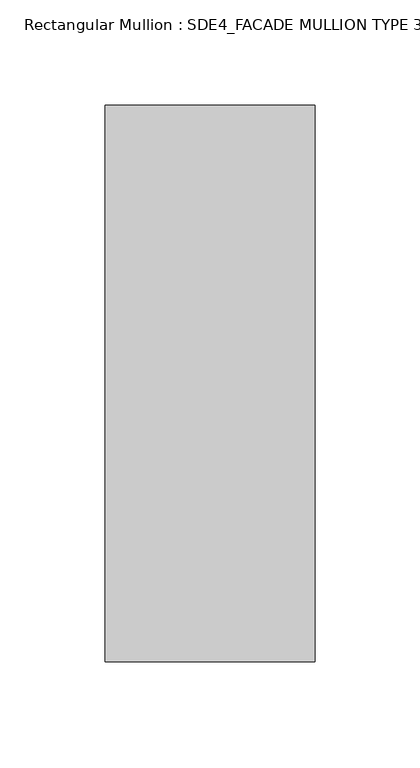
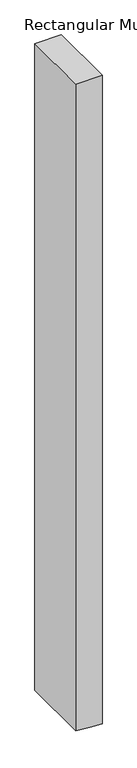
"""IFC4 building model written with IfcOpenShell, lengths in millimetres: member geometry, Rectangular Mullion : SDE4_FACADE MULLION TYPE 3."""

import ifcopenshell
import ifcopenshell.guid

model = None  # the IFC model being written
_history = None  # IfcOwnerHistory: only IFC2X3 demands one
_inside = {}  # id of a spatial element -> (the spatial element, [elements in it])
_under = {}  # id of a project, library or spatial element -> (it, [spatial elements below it])
_declared = {}  # id of a project -> (the project, [libraries it declares])
_typed = {}  # id of a type object -> (the type object, [elements of that type])
_made_of = {}  # id of a material, layer set ... -> (it, [elements and type objects made of it])


def new_model(schema):
    """Start an empty IFC model of exactly this schema.

    Asked for "IFC4X3", IfcOpenShell would pick the latest addendum, in which some entities
    have other attributes; the version numbers below select the first issue.
    IFC2X3 requires an IfcOwnerHistory on every rooted entity: one is made here for all.
    """
    global model, _history
    if schema == "IFC4X3":
        model = ifcopenshell.file(schema_version=(4, 3, 0, 0))
    else:
        model = ifcopenshell.file(schema=schema)
    _inside.clear()
    _under.clear()
    _declared.clear()
    _typed.clear()
    _made_of.clear()
    _history = None
    if model.schema == "IFC2X3":
        org = make("IfcOrganization", Name="unknown")
        user = make(
            "IfcPersonAndOrganization",
            ThePerson=make("IfcPerson", FamilyName="unknown"),
            TheOrganization=org,
        )
        app = make(
            "IfcApplication",
            ApplicationDeveloper=org,
            Version="unknown",
            ApplicationFullName="unknown",
            ApplicationIdentifier="unknown",
        )
        _history = make(
            "IfcOwnerHistory",
            OwningUser=user,
            OwningApplication=app,
            ChangeAction="ADDED",
            CreationDate=0,
        )
    return model


def make(cls, **values):
    """One entity of the class cls with the attributes given. An attribute that is None is left unset."""
    return model.create_entity(
        cls, **{name: value for name, value in values.items() if value is not None}
    )


def rooted(cls, **values):
    """An entity with a GlobalId (a new one), such as an element, a storey or a relation."""
    return make(cls, GlobalId=ifcopenshell.guid.new(), OwnerHistory=_history, **values)


def si_unit(unit_type, name, prefix=None):
    """IfcSIUnit, for example si_unit("LENGTHUNIT", "METRE", prefix="MILLI")."""
    return make("IfcSIUnit", UnitType=unit_type, Prefix=prefix, Name=name)


def assignment(units):
    """IfcUnitAssignment: the units of a project."""
    return None if units is None else make("IfcUnitAssignment", Units=units)


def point(xyz):
    """IfcCartesianPoint."""
    return None if xyz is None else make("IfcCartesianPoint", Coordinates=xyz)


def direction(xyz):
    """IfcDirection."""
    return None if xyz is None else make("IfcDirection", DirectionRatios=xyz)


def frame(location, z_axis=None, x_axis=None):
    """IfcAxis2Placement3D, a coordinate frame: its origin and axes. An axis left out is left unset."""
    return make(
        "IfcAxis2Placement3D",
        Location=point(location),
        Axis=direction(z_axis),
        RefDirection=direction(x_axis),
    )


def origin():
    """The frame at (0, 0, 0) with its axes left unset."""
    return frame((0.0, 0.0, 0.0))


def place(relative_to, where):
    """IfcLocalPlacement: puts the frame where relative to a parent placement (None: the world)."""
    return make(
        "IfcLocalPlacement", PlacementRelTo=relative_to, RelativePlacement=where
    )


def context(
    kind, dimensions, precision=None, world=None, true_north=None, identifier=None
):
    """IfcGeometricRepresentationContext, for example the 3D "Model" context."""
    return make(
        "IfcGeometricRepresentationContext",
        ContextIdentifier=identifier,
        ContextType=kind,
        CoordinateSpaceDimension=dimensions,
        Precision=precision,
        WorldCoordinateSystem=world,
        TrueNorth=true_north,
    )


def project(units=None, contexts=None):
    """IfcProject with its units and contexts."""
    return rooted(
        "IfcProject",
        Name="project",
        RepresentationContexts=contexts,
        UnitsInContext=assignment(units),
    )


def spatial(cls, under=None, at=None, **own):
    """A site, building, storey or space (cls), placed at a placement, below another one or the project."""
    s = rooted(cls, ObjectPlacement=at, **own)
    if under is not None:
        _under.setdefault(under.id(), (under, []))[1].append(s)
    return s


def polyline(points):
    """IfcPolyline through the points."""
    return make("IfcPolyline", Points=[point(p) for p in points])


def outline(outer, holes=None, kind="AREA"):
    """IfcArbitraryClosedProfileDef: a profile drawn as a closed curve; with holes, ...WithVoids."""
    if holes is None:
        return make("IfcArbitraryClosedProfileDef", ProfileType=kind, OuterCurve=outer)
    return make(
        "IfcArbitraryProfileDefWithVoids",
        ProfileType=kind,
        OuterCurve=outer,
        InnerCurves=holes,
    )


def extrude(swept, where, along, depth):
    """IfcExtrudedAreaSolid: the profile swept, set in the frame where, extruded along a direction by depth."""
    return make(
        "IfcExtrudedAreaSolid",
        SweptArea=swept,
        Position=where,
        ExtrudedDirection=direction(along),
        Depth=depth,
    )


def shape(context_of_items, identifier, shape_type, items):
    """IfcShapeRepresentation: the items that make up one representation, for example the "Body"."""
    return make(
        "IfcShapeRepresentation",
        ContextOfItems=context_of_items,
        RepresentationIdentifier=identifier,
        RepresentationType=shape_type,
        Items=items,
    )


def source(mapping_origin, context_of_items, identifier, shape_type, items):
    """IfcRepresentationMap: a shape defined once, which mapped items show again and again."""
    return make(
        "IfcRepresentationMap",
        MappingOrigin=mapping_origin,
        MappedRepresentation=shape(context_of_items, identifier, shape_type, items),
    )


def transform(
    local_origin,
    x_axis=None,
    y_axis=None,
    z_axis=None,
    scale=None,
    scale2=None,
    scale3=None,
    uniform=True,
):
    """IfcCartesianTransformationOperator3D, or its non-uniform kind. x_axis, y_axis, z_axis: its Axis1, 2, 3."""
    if uniform:
        return make(
            "IfcCartesianTransformationOperator3D",
            Axis1=direction(x_axis),
            Axis2=direction(y_axis),
            LocalOrigin=point(local_origin),
            Scale=scale,
            Axis3=direction(z_axis),
        )
    return make(
        "IfcCartesianTransformationOperator3DnonUniform",
        Axis1=direction(x_axis),
        Axis2=direction(y_axis),
        LocalOrigin=point(local_origin),
        Scale=scale,
        Axis3=direction(z_axis),
        Scale2=scale2,
        Scale3=scale3,
    )


def mapped(mapping_source, mapping_target):
    """IfcMappedItem: shows the shape of a source again, moved by a transform."""
    return make(
        "IfcMappedItem", MappingSource=mapping_source, MappingTarget=mapping_target
    )


def made_of(thing, what):
    """Note that an element or type object is made of a material, layer set ...; save() writes the relation."""
    if what is not None:
        _made_of.setdefault(what.id(), (what, []))[1].append(thing)
    return thing


def element(
    cls,
    number,
    at=None,
    inside=None,
    cuts=None,
    type_object=None,
    material=None,
    context=None,
    identifier="Body",
    shape_type=None,
    held_by="IfcProductDefinitionShape",
    body=None,
    shapes=None,
    **own,
):
    """One element of the class cls, such as IfcWall. Its Tag is "e" and its number.

    at: its placement. inside: the storey or other place that contains it. cuts: it is an
    opening in that element (IfcRelVoidsElement). A single representation is given by context,
    identifier, shape_type and body (its items); several are given by shapes. held_by: the class
    of the entity that holds the representations. save() writes the other relations.
    """
    e = rooted(cls, Tag="e%d" % number, ObjectPlacement=at, **own)
    if body is not None:
        shapes = [shape(context, identifier, shape_type, body)]
    if shapes is not None:
        e.Representation = make(held_by, Representations=shapes)
    if inside is not None:
        _inside.setdefault(inside.id(), (inside, []))[1].append(e)
    if cuts is not None:
        rooted(
            "IfcRelVoidsElement", RelatingBuildingElement=cuts, RelatedOpeningElement=e
        )
    if type_object is not None:
        _typed.setdefault(type_object.id(), (type_object, []))[1].append(e)
    return made_of(e, material)


def aggregate(whole, parts):
    """IfcRelAggregates: a whole, such as a stair, and the parts it consists of."""
    return rooted("IfcRelAggregates", RelatingObject=whole, RelatedObjects=parts)


def save(model, path):
    """Write the relations noted so far, then the file.

    IfcRelAggregates (storeys below a building ...), IfcRelContainedInSpatialStructure (elements
    in a storey), IfcRelDefinesByType, IfcRelAssociatesMaterial and IfcRelDeclares: one each for
    every whole, place, type object, material and project.
    """
    for whole, parts in _under.values():
        aggregate(whole, parts)
    for where, things in _inside.values():
        rooted(
            "IfcRelContainedInSpatialStructure",
            RelatedElements=things,
            RelatingStructure=where,
        )
    for kind, things in _typed.values():
        rooted("IfcRelDefinesByType", RelatedObjects=things, RelatingType=kind)
    for what, things in _made_of.values():
        rooted("IfcRelAssociatesMaterial", RelatedObjects=things, RelatingMaterial=what)
    for by, libraries in _declared.values():
        rooted("IfcRelDeclares", RelatingContext=by, RelatedDefinitions=libraries)
    model.write(path)


def rectangular_mullion_sde4_facade_mullion_type_3_52749065(model_context):
    return source(origin(), model_context, "Body", "SweptSolid", [
        extrude(outline(polyline([(0.0, 50.0), (0.0, -50.0), (-2578.6532532, -50.0), (-2582.7193322, 3.056508), (-2586.3169295, 50.0), (0.0, 50.0)])), frame((0.0, -132.5, 0.0), z_axis=(0.0, 1.0, 0.0), x_axis=(0.0, 0.0, 1.0)), (0.0, 0.0, 1.0), 265.0),
    ])


if __name__ == "__main__":
    model = new_model("IFC4")
    model_context = context("Model", 3, world=origin())
    ifc_project = project(units=[si_unit("LENGTHUNIT", "METRE", prefix="MILLI")], contexts=[model_context])
    site = spatial("IfcSite", under=ifc_project)
    building = spatial("IfcBuilding", under=site)
    placement = place(None, origin())
    rectangular_mullion_sde4_facade_mullion_type_3_shape = rectangular_mullion_sde4_facade_mullion_type_3_52749065(model_context)
    element("IfcMember", 1, ObjectType="Rectangular Mullion : SDE4_FACADE MULLION TYPE 3", at=placement, inside=building, context=model_context, shape_type="MappedRepresentation", body=[
        mapped(rectangular_mullion_sde4_facade_mullion_type_3_shape, transform((0.0, 0.0, 0.0), x_axis=(1.0, 0.0, 0.0), y_axis=(0.0, 1.0, 0.0), z_axis=(0.0, 0.0, 1.0))),
    ])
    save(model, "model.ifc")

# Revit data of these elements
# Type "Rectangular Mullion : SDE4_FACADE MULLION TYPE 3"
#   built-in parameter 1007322 = 0.869423 (stored number, unit not read)
#   built-in parameter 1007321 = 0.164042 (stored number, unit not read)
#   built-in parameter 1007320 = 0.164042 (stored number, unit not read)
